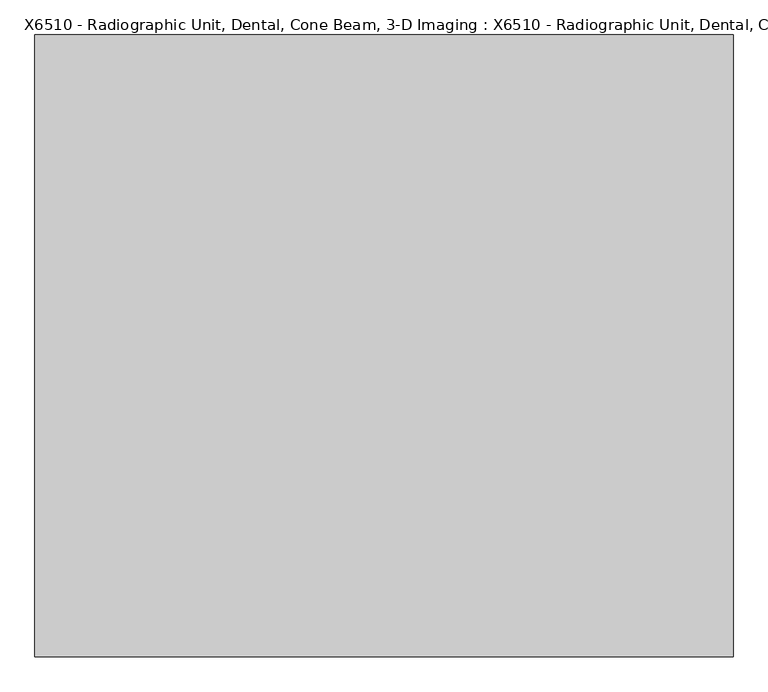
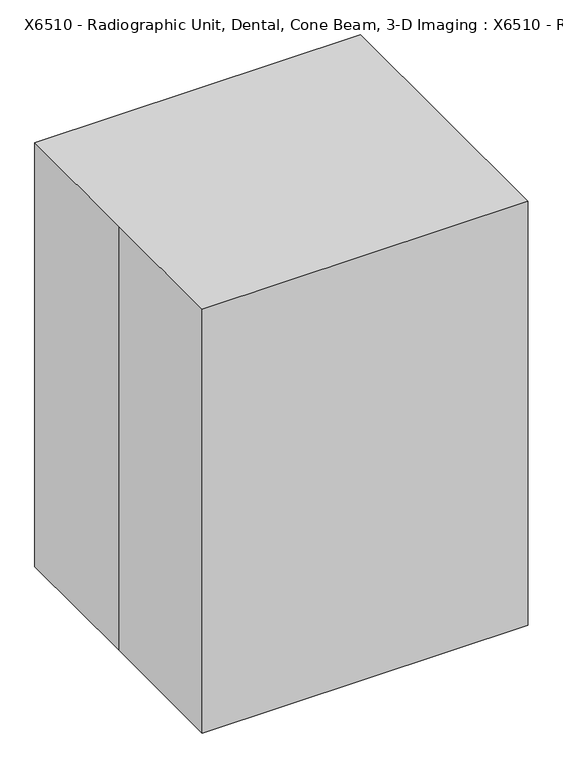
"""IFC4 building model written with IfcOpenShell, lengths in millimetres: proxy geometry, X6510 - Radiographic Unit, Dental, Cone Beam, 3-D Imaging : X6510 - Radiographic Unit, Dental, Cone Beam, 3-D Imaging."""

import ifcopenshell
import ifcopenshell.guid

model = None  # the IFC model being written
_history = None  # IfcOwnerHistory: only IFC2X3 demands one
_inside = {}  # id of a spatial element -> (the spatial element, [elements in it])
_under = {}  # id of a project, library or spatial element -> (it, [spatial elements below it])
_declared = {}  # id of a project -> (the project, [libraries it declares])
_typed = {}  # id of a type object -> (the type object, [elements of that type])
_made_of = {}  # id of a material, layer set ... -> (it, [elements and type objects made of it])


def new_model(schema):
    """Start an empty IFC model of exactly this schema.

    Asked for "IFC4X3", IfcOpenShell would pick the latest addendum, in which some entities
    have other attributes; the version numbers below select the first issue.
    IFC2X3 requires an IfcOwnerHistory on every rooted entity: one is made here for all.
    """
    global model, _history
    if schema == "IFC4X3":
        model = ifcopenshell.file(schema_version=(4, 3, 0, 0))
    else:
        model = ifcopenshell.file(schema=schema)
    _inside.clear()
    _under.clear()
    _declared.clear()
    _typed.clear()
    _made_of.clear()
    _history = None
    if model.schema == "IFC2X3":
        org = make("IfcOrganization", Name="unknown")
        user = make(
            "IfcPersonAndOrganization",
            ThePerson=make("IfcPerson", FamilyName="unknown"),
            TheOrganization=org,
        )
        app = make(
            "IfcApplication",
            ApplicationDeveloper=org,
            Version="unknown",
            ApplicationFullName="unknown",
            ApplicationIdentifier="unknown",
        )
        _history = make(
            "IfcOwnerHistory",
            OwningUser=user,
            OwningApplication=app,
            ChangeAction="ADDED",
            CreationDate=0,
        )
    return model


def make(cls, **values):
    """One entity of the class cls with the attributes given. An attribute that is None is left unset."""
    return model.create_entity(
        cls, **{name: value for name, value in values.items() if value is not None}
    )


def rooted(cls, **values):
    """An entity with a GlobalId (a new one), such as an element, a storey or a relation."""
    return make(cls, GlobalId=ifcopenshell.guid.new(), OwnerHistory=_history, **values)


def si_unit(unit_type, name, prefix=None):
    """IfcSIUnit, for example si_unit("LENGTHUNIT", "METRE", prefix="MILLI")."""
    return make("IfcSIUnit", UnitType=unit_type, Prefix=prefix, Name=name)


def assignment(units):
    """IfcUnitAssignment: the units of a project."""
    return None if units is None else make("IfcUnitAssignment", Units=units)


def point(xyz):
    """IfcCartesianPoint."""
    return None if xyz is None else make("IfcCartesianPoint", Coordinates=xyz)


def direction(xyz):
    """IfcDirection."""
    return None if xyz is None else make("IfcDirection", DirectionRatios=xyz)


def frame(location, z_axis=None, x_axis=None):
    """IfcAxis2Placement3D, a coordinate frame: its origin and axes. An axis left out is left unset."""
    return make(
        "IfcAxis2Placement3D",
        Location=point(location),
        Axis=direction(z_axis),
        RefDirection=direction(x_axis),
    )


def frame_2d(location, x_axis=None):
    """IfcAxis2Placement2D, a coordinate frame in the plane: its origin and x axis."""
    return make(
        "IfcAxis2Placement2D", Location=point(location), RefDirection=direction(x_axis)
    )


def origin():
    """The frame at (0, 0, 0) with its axes left unset."""
    return frame((0.0, 0.0, 0.0))


def origin_with_axes():
    """The frame at (0, 0, 0) with the z axis (0, 0, 1) and the x axis (1, 0, 0) written out."""
    return frame((0.0, 0.0, 0.0), z_axis=(0.0, 0.0, 1.0), x_axis=(1.0, 0.0, 0.0))


def place(relative_to, where):
    """IfcLocalPlacement: puts the frame where relative to a parent placement (None: the world)."""
    return make(
        "IfcLocalPlacement", PlacementRelTo=relative_to, RelativePlacement=where
    )


def context(
    kind, dimensions, precision=None, world=None, true_north=None, identifier=None
):
    """IfcGeometricRepresentationContext, for example the 3D "Model" context."""
    return make(
        "IfcGeometricRepresentationContext",
        ContextIdentifier=identifier,
        ContextType=kind,
        CoordinateSpaceDimension=dimensions,
        Precision=precision,
        WorldCoordinateSystem=world,
        TrueNorth=true_north,
    )


def project(units=None, contexts=None):
    """IfcProject with its units and contexts."""
    return rooted(
        "IfcProject",
        Name="project",
        RepresentationContexts=contexts,
        UnitsInContext=assignment(units),
    )


def spatial(cls, under=None, at=None, **own):
    """A site, building, storey or space (cls), placed at a placement, below another one or the project."""
    s = rooted(cls, ObjectPlacement=at, **own)
    if under is not None:
        _under.setdefault(under.id(), (under, []))[1].append(s)
    return s


def polyline(points):
    """IfcPolyline through the points."""
    return make("IfcPolyline", Points=[point(p) for p in points])


def circle_curve(where, radius):
    """IfcCircle in the frame where."""
    return make("IfcCircle", Position=where, Radius=radius)


def trimmed(basis, trim1, trim2, sense, master):
    """IfcTrimmedCurve: the piece of a basis curve between two trims."""
    return make(
        "IfcTrimmedCurve",
        BasisCurve=basis,
        Trim1=trim1,
        Trim2=trim2,
        SenseAgreement=sense,
        MasterRepresentation=master,
    )


def segment(curve, same_sense, transition):
    """IfcCompositeCurveSegment."""
    return make(
        "IfcCompositeCurveSegment",
        Transition=transition,
        SameSense=same_sense,
        ParentCurve=curve,
    )


def composite_curve(segments, self_intersect=None):
    """IfcCompositeCurve: segments joined end to end."""
    return make("IfcCompositeCurve", Segments=segments, SelfIntersect=self_intersect)


def outline(outer, holes=None, kind="AREA"):
    """IfcArbitraryClosedProfileDef: a profile drawn as a closed curve; with holes, ...WithVoids."""
    if holes is None:
        return make("IfcArbitraryClosedProfileDef", ProfileType=kind, OuterCurve=outer)
    return make(
        "IfcArbitraryProfileDefWithVoids",
        ProfileType=kind,
        OuterCurve=outer,
        InnerCurves=holes,
    )


def extrude(swept, where, along, depth):
    """IfcExtrudedAreaSolid: the profile swept, set in the frame where, extruded along a direction by depth."""
    return make(
        "IfcExtrudedAreaSolid",
        SweptArea=swept,
        Position=where,
        ExtrudedDirection=direction(along),
        Depth=depth,
    )


def shape(context_of_items, identifier, shape_type, items):
    """IfcShapeRepresentation: the items that make up one representation, for example the "Body"."""
    return make(
        "IfcShapeRepresentation",
        ContextOfItems=context_of_items,
        RepresentationIdentifier=identifier,
        RepresentationType=shape_type,
        Items=items,
    )


def source(mapping_origin, context_of_items, identifier, shape_type, items):
    """IfcRepresentationMap: a shape defined once, which mapped items show again and again."""
    return make(
        "IfcRepresentationMap",
        MappingOrigin=mapping_origin,
        MappedRepresentation=shape(context_of_items, identifier, shape_type, items),
    )


def transform(
    local_origin,
    x_axis=None,
    y_axis=None,
    z_axis=None,
    scale=None,
    scale2=None,
    scale3=None,
    uniform=True,
):
    """IfcCartesianTransformationOperator3D, or its non-uniform kind. x_axis, y_axis, z_axis: its Axis1, 2, 3."""
    if uniform:
        return make(
            "IfcCartesianTransformationOperator3D",
            Axis1=direction(x_axis),
            Axis2=direction(y_axis),
            LocalOrigin=point(local_origin),
            Scale=scale,
            Axis3=direction(z_axis),
        )
    return make(
        "IfcCartesianTransformationOperator3DnonUniform",
        Axis1=direction(x_axis),
        Axis2=direction(y_axis),
        LocalOrigin=point(local_origin),
        Scale=scale,
        Axis3=direction(z_axis),
        Scale2=scale2,
        Scale3=scale3,
    )


def mapped(mapping_source, mapping_target):
    """IfcMappedItem: shows the shape of a source again, moved by a transform."""
    return make(
        "IfcMappedItem", MappingSource=mapping_source, MappingTarget=mapping_target
    )


def made_of(thing, what):
    """Note that an element or type object is made of a material, layer set ...; save() writes the relation."""
    if what is not None:
        _made_of.setdefault(what.id(), (what, []))[1].append(thing)
    return thing


def element(
    cls,
    number,
    at=None,
    inside=None,
    cuts=None,
    type_object=None,
    material=None,
    context=None,
    identifier="Body",
    shape_type=None,
    held_by="IfcProductDefinitionShape",
    body=None,
    shapes=None,
    **own,
):
    """One element of the class cls, such as IfcWall. Its Tag is "e" and its number.

    at: its placement. inside: the storey or other place that contains it. cuts: it is an
    opening in that element (IfcRelVoidsElement). A single representation is given by context,
    identifier, shape_type and body (its items); several are given by shapes. held_by: the class
    of the entity that holds the representations. save() writes the other relations.
    """
    e = rooted(cls, Tag="e%d" % number, ObjectPlacement=at, **own)
    if body is not None:
        shapes = [shape(context, identifier, shape_type, body)]
    if shapes is not None:
        e.Representation = make(held_by, Representations=shapes)
    if inside is not None:
        _inside.setdefault(inside.id(), (inside, []))[1].append(e)
    if cuts is not None:
        rooted(
            "IfcRelVoidsElement", RelatingBuildingElement=cuts, RelatedOpeningElement=e
        )
    if type_object is not None:
        _typed.setdefault(type_object.id(), (type_object, []))[1].append(e)
    return made_of(e, material)


def aggregate(whole, parts):
    """IfcRelAggregates: a whole, such as a stair, and the parts it consists of."""
    return rooted("IfcRelAggregates", RelatingObject=whole, RelatedObjects=parts)


def save(model, path):
    """Write the relations noted so far, then the file.

    IfcRelAggregates (storeys below a building ...), IfcRelContainedInSpatialStructure (elements
    in a storey), IfcRelDefinesByType, IfcRelAssociatesMaterial and IfcRelDeclares: one each for
    every whole, place, type object, material and project.
    """
    for whole, parts in _under.values():
        aggregate(whole, parts)
    for where, things in _inside.values():
        rooted(
            "IfcRelContainedInSpatialStructure",
            RelatedElements=things,
            RelatingStructure=where,
        )
    for kind, things in _typed.values():
        rooted("IfcRelDefinesByType", RelatedObjects=things, RelatingType=kind)
    for what, things in _made_of.values():
        rooted("IfcRelAssociatesMaterial", RelatedObjects=things, RelatingMaterial=what)
    for by, libraries in _declared.values():
        rooted("IfcRelDeclares", RelatingContext=by, RelatedDefinitions=libraries)
    model.write(path)


def x6510_radiographic_unit_dental_cone_beam_3_d_imaging_x6510_5ab47b50(model_context):
    return source(origin(), model_context, "Body", "SweptSolid", [
        extrude(outline(polyline([(178.0903289, 963.09198), (178.0903289, 658.29198), (101.8903289, 658.29198), (101.8903289, 886.89198), (-228.3096711, 886.89198), (-228.3096711, 963.09198), (178.0903289, 963.09198)])), frame((-292.7334291, 0.0, 0.0), z_axis=(1.0, 0.0, 0.0), x_axis=(0.0, 1.0, 0.0)), (0.0, 0.0, 1.0), 52.0668582),
        extrude(outline(polyline([(178.0903289, 963.09198), (178.0903289, 658.29198), (101.8903289, 658.29198), (101.8903289, 886.89198), (-228.3096711, 886.89198), (-228.3096711, 963.09198), (178.0903289, 963.09198)])), frame((240.6665709, 0.0, 0.0), z_axis=(1.0, 0.0, 0.0), x_axis=(0.0, 1.0, 0.0)), (0.0, 0.0, 1.0), 55.7916128),
        extrude(outline(composite_curve([segment(trimmed(circle_curve(frame_2d((-0.6135895, 76.2)), 152.4), [point((-153.0135895, 76.2))], [point((151.7864105, 76.2))], False, "CARTESIAN"), True, "CONTINUOUS"), segment(trimmed(circle_curve(frame_2d((-0.6135895, 76.2)), 152.4), [point((151.7864105, 76.2))], [point((-153.0135895, 76.2))], False, "CARTESIAN"), True, "CONTINUOUS")], self_intersect=False)), frame((0.0, 0.0, 101.6), z_axis=(0.0, 0.0, 1.0), x_axis=(1.0, 0.0, 0.0)), (0.0, 0.0, 1.0), 556.69198),
        extrude(outline(polyline([(-389.0886204, 132.4077326), (-587.7516592, 193.1451188), (-572.8991766, 241.7254004), (-455.5928432, 205.8612552), (-288.6985003, 751.7480536), (314.8123695, 751.7480536), (426.4735529, 1235.4057755), (521.5656481, 1213.4520355), (393.3968503, 658.29198), (-228.3096711, 658.29198), (-389.0886204, 132.4077326)])), frame((-240.6665709, 0.0, 0.0), z_axis=(1.0, 0.0, 0.0), x_axis=(0.0, 1.0, 0.0)), (0.0, 0.0, 1.0), 481.3331418),
        extrude(outline(polyline([(1905.6637062, 570.8864105), (1905.6637062, -572.1135895), (1448.4637062, -572.1135895), (1448.4637062, -368.9135895), (1473.8637062, -368.9135895), (1527.7452429, -315.0320528), (1603.9452429, -315.0320528), (1657.8267796, -368.9135895), (1804.0637062, -368.9135895), (1804.0637062, 418.4864105), (1448.4637062, 418.4864105), (1448.4637062, 570.8864105), (1905.6637062, 570.8864105)])), frame((0.0, 0.0, 0.0), z_axis=(0.0, 1.0, 0.0), x_axis=(0.0, 0.0, 1.0)), (0.0, 0.0, 1.0), 410.7434845),
        extrude(outline(polyline([(-657.225, -184.15), (-657.225, 120.65), (657.225, 120.65), (657.225, -184.15), (-657.225, -184.15)])), origin_with_axes(), (0.0, 0.0, 1.0), 101.6),
        extrude(outline(polyline([(2079.625, 809.625), (2079.625, -809.625), (0.0, -809.625), (0.0, 809.625), (2079.625, 809.625)]), holes=[polyline([(1978.025, 657.225), (101.6, 657.225), (101.6, -657.225), (1978.025, -657.225), (1978.025, 657.225)])]), frame((0.0, 120.65, 0.0), z_axis=(0.0, 1.0, 0.0), x_axis=(0.0, 0.0, 1.0)), (0.0, 0.0, 1.0), 304.8),
        extrude(outline(polyline([(-812.8, 723.9), (812.8, 723.9), (812.8, -723.9), (-812.8, -723.9), (-812.8, 0.0), (-812.8, 723.9)])), origin_with_axes(), (0.0, 0.0, 1.0), 2235.2),
    ])


if __name__ == "__main__":
    model = new_model("IFC4")
    model_context = context("Model", 3, world=origin())
    ifc_project = project(units=[si_unit("LENGTHUNIT", "METRE", prefix="MILLI")], contexts=[model_context])
    site = spatial("IfcSite", under=ifc_project)
    building = spatial("IfcBuilding", under=site)
    placement = place(None, origin())
    x6510_radiographic_unit_dental_cone_beam_3_d_imaging_x6510_shape = x6510_radiographic_unit_dental_cone_beam_3_d_imaging_x6510_5ab47b50(model_context)
    element("IfcBuildingElementProxy", 1, Name="X6510 - Radiographic Unit, Dental, Cone Beam, 3-D Imaging : X6510 - Radiographic Unit, Dental, Cone Beam, 3-D Imaging", ObjectType="X6510 - Radiographic Unit, Dental, Cone Beam, 3-D Imaging : X6510 - Radiographic Unit, Dental, Cone Beam, 3-D Imaging", at=placement, inside=building, context=model_context, shape_type="MappedRepresentation", body=[
        mapped(x6510_radiographic_unit_dental_cone_beam_3_d_imaging_x6510_shape, transform((0.0, 0.0, 0.0), x_axis=(1.0, 0.0, 0.0), y_axis=(0.0, 1.0, 0.0), z_axis=(0.0, 0.0, 1.0))),
    ])
    save(model, "model.ifc")

# Revit data of these elements
# Project information
#   Sheets - Total = "5"
#   Project Issue Date = "Issue Date"
#   Project Status = "Project Status"
#   Client Name = "Owner"
#   Project Address = "Enter address here"
#   Project Name = "Project Name"
#   Project Number = "Project Number"
#   Publication Date = "30-Jan-15"
# Type "X6510 - Radiographic Unit, Dental, Cone Beam, 3-D Imaging : X6510 - Radiographic Unit, Dental, Cone Beam, 3-D Imaging"
#   Watts2 = "0"
#   Watts1 = "1200"
#   Unit_Issue = "EA"
#   UTIL_6_Misc = "-"
#   UTIL_5_NonMedGas = "-"
#   UTIL_4_MiscGas = "-"
#   UTIL_3_MedGas = "-"
#   UTIL_2_Elec = "F"
#   UTIL_1_WaterDrain = "-"
#   Nomenclature = "Radiographic Unit, Dental, Cone Beam, 3-D Imaging"
#   NSN = "6525"
#   Location [instance default] = ""
#   JSN = "X6510"
#   Fund_Source_VA = "-"
#   Fund_Source_Navy = "-"
#   Fund_Source_Army = "-"
#   Fund_Source_AF = "-"
#   ELEC_Volts2 = "0"
#   ELEC_Volts1 = "120"
#   ELEC_Phase2 = "0"
#   ELEC_Phase1 = "1"
#   ELEC_HertzSwitch = "-1"
#   ELEC_HertzDependent = "0"
#   ELEC_Hertz = "0"
#   ELEC_Amps2 = "0"
#   ELEC_Amps1 = "10"
#   DetailDescription = "x6510A dental radiographic unit providing three-dimensional images. The unit uses a cone-shaped beam to acquire an image in a single pass. The unit provides a superior high resolution 3D image with low radiation dosage. Allows comprehensive examination and precise information on the anatomy of a patients mouth, face and jaw areas by producing 3D images of all oral and maxillofacial structures."
#   CAT_VA = "F"
#   CAT_Navy = "F"
#   CAT_IHS = "-"
#   CAT_Army = "F"
#   CAT_AF = "F"
#   BTUperhour = "0"
#   Weight_IP = 882
#   DIM_Width_IP = 5' - 4"
#   DIM_Height_IP = 7' - 4"
#   DIM_Depth_IP = 4' - 9"
# Element 1 (IfcBuildingElementProxy, "X6510 - Radiographic Unit, Dental, Cone Beam, 3-D Imaging : X6510 - Radiographic Unit, Dental, Cone Beam, 3-D Imaging")
#   Materials on its faces: "EquipSpace"
# Materials
#   "EquipSpace": class "Unassigned", colour RGB 221 217 195, transparency 0.5
